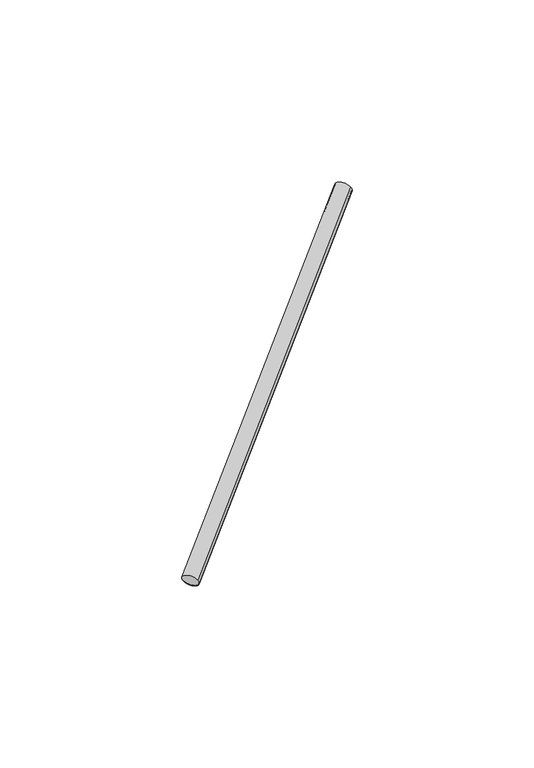
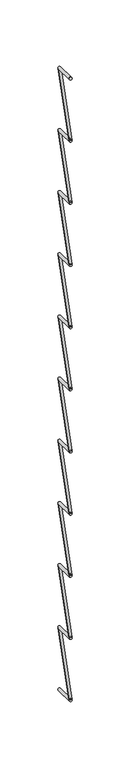
"""IFC4 building model written with IfcOpenShell, lengths in millimetres: proxy geometry, Pre-fab. (Vigota 2 - Pano 4)."""

from ifc_helpers import new_model, si_unit, point, frame, origin, origin_2d, place, context, project, spatial, circle_curve, trimmed, segment, composite_curve, outline, extrude, source, transform, mapped, element, save


def structural_framing_d21f35b0(model_context):
    return source(origin(), model_context, "Body", "SweptSolid", [
        extrude(outline(composite_curve([segment(trimmed(circle_curve(origin_2d(), 2.5), [point((2.5, 0.0))], [point((-2.5, 0.0))], False, "CARTESIAN"), True, "CONTINUOUS"), segment(trimmed(circle_curve(origin_2d(), 2.5), [point((-2.5, 0.0))], [point((2.5, 0.0))], False, "CARTESIAN"), True, "CONTINUOUS")], self_intersect=False)), frame((-42.0, 108.0, 1797.0), z_axis=(-0.3218603428886276, -0.8276408817707567, 0.4598004898837537), x_axis=(0.8192319205108605, 3.936835275445103e-11, 0.5734623443750141)), (0.0, 0.0, 1.0), 130.491379),
        extrude(outline(composite_curve([segment(trimmed(circle_curve(origin_2d(), 2.5), [point((2.5, 0.0))], [point((-2.5, 0.0))], False, "CARTESIAN"), True, "CONTINUOUS"), segment(trimmed(circle_curve(origin_2d(), 2.5), [point((-2.5, 0.0))], [point((2.5, 0.0))], False, "CARTESIAN"), True, "CONTINUOUS")], self_intersect=False)), frame((-84.0, 0.0, 1857.0), z_axis=(0.3218603428886276, 0.8276408817707567, 0.4598004898837537), x_axis=(0.8192319205108605, 3.936835275445103e-11, -0.5734623443750141)), (0.0, 0.0, 1.0), 130.491379),
        extrude(outline(composite_curve([segment(trimmed(circle_curve(origin_2d(), 2.5), [point((2.5, 0.0))], [point((-2.5, 0.0))], False, "CARTESIAN"), True, "CONTINUOUS"), segment(trimmed(circle_curve(origin_2d(), 2.5), [point((-2.5, 0.0))], [point((2.5, 0.0))], False, "CARTESIAN"), True, "CONTINUOUS")], self_intersect=False)), frame((-42.0, 108.0, 1917.0), z_axis=(-0.3218603428886276, -0.8276408817707567, 0.4598004898837537), x_axis=(0.8192319205108605, 3.936835275445103e-11, 0.5734623443750141)), (0.0, 0.0, 1.0), 130.491379),
        extrude(outline(composite_curve([segment(trimmed(circle_curve(origin_2d(), 2.5), [point((2.5, 0.0))], [point((-2.5, 0.0))], False, "CARTESIAN"), True, "CONTINUOUS"), segment(trimmed(circle_curve(origin_2d(), 2.5), [point((-2.5, 0.0))], [point((2.5, 0.0))], False, "CARTESIAN"), True, "CONTINUOUS")], self_intersect=False)), frame((-84.0, 0.0, 1977.0), z_axis=(0.3218603428886276, 0.8276408817707567, 0.4598004898837537), x_axis=(0.8192319205108605, 3.936835275445103e-11, -0.5734623443750141)), (0.0, 0.0, 1.0), 130.491379),
        extrude(outline(composite_curve([segment(trimmed(circle_curve(origin_2d(), 2.5), [point((2.5, 0.0))], [point((-2.5, 0.0))], False, "CARTESIAN"), True, "CONTINUOUS"), segment(trimmed(circle_curve(origin_2d(), 2.5), [point((-2.5, 0.0))], [point((2.5, 0.0))], False, "CARTESIAN"), True, "CONTINUOUS")], self_intersect=False)), frame((-42.0, 108.0, 2037.0), z_axis=(-0.3218603428886276, -0.8276408817707567, 0.4598004898837537), x_axis=(0.8192319205108605, 3.936835275445103e-11, 0.5734623443750141)), (0.0, 0.0, 1.0), 130.491379),
        extrude(outline(composite_curve([segment(trimmed(circle_curve(origin_2d(), 2.5), [point((2.5, 0.0))], [point((-2.5, 0.0))], False, "CARTESIAN"), True, "CONTINUOUS"), segment(trimmed(circle_curve(origin_2d(), 2.5), [point((-2.5, 0.0))], [point((2.5, 0.0))], False, "CARTESIAN"), True, "CONTINUOUS")], self_intersect=False)), frame((-84.0, 0.0, 2097.0), z_axis=(0.3218603428886276, 0.8276408817707567, 0.4598004898837537), x_axis=(0.8192319205108605, 3.936835275445103e-11, -0.5734623443750141)), (0.0, 0.0, 1.0), 130.491379),
        extrude(outline(composite_curve([segment(trimmed(circle_curve(origin_2d(), 2.5), [point((2.5, 0.0))], [point((-2.5, 0.0))], False, "CARTESIAN"), True, "CONTINUOUS"), segment(trimmed(circle_curve(origin_2d(), 2.5), [point((-2.5, 0.0))], [point((2.5, 0.0))], False, "CARTESIAN"), True, "CONTINUOUS")], self_intersect=False)), frame((-42.0, 108.0, 2157.0), z_axis=(-0.3218603428886276, -0.8276408817707567, 0.4598004898837537), x_axis=(0.8192319205108605, 3.936835275445103e-11, 0.5734623443750141)), (0.0, 0.0, 1.0), 130.491379),
        extrude(outline(composite_curve([segment(trimmed(circle_curve(origin_2d(), 2.5), [point((2.5, 0.0))], [point((-2.5, 0.0))], False, "CARTESIAN"), True, "CONTINUOUS"), segment(trimmed(circle_curve(origin_2d(), 2.5), [point((-2.5, 0.0))], [point((2.5, 0.0))], False, "CARTESIAN"), True, "CONTINUOUS")], self_intersect=False)), frame((-84.0, 0.0, 2217.0), z_axis=(0.3218603428886276, 0.8276408817707567, 0.4598004898837537), x_axis=(0.8192319205108605, 3.936835275445103e-11, -0.5734623443750141)), (0.0, 0.0, 1.0), 130.491379),
        extrude(outline(composite_curve([segment(trimmed(circle_curve(origin_2d(), 2.5), [point((2.5, 0.0))], [point((-2.5, 0.0))], False, "CARTESIAN"), True, "CONTINUOUS"), segment(trimmed(circle_curve(origin_2d(), 2.5), [point((-2.5, 0.0))], [point((2.5, 0.0))], False, "CARTESIAN"), True, "CONTINUOUS")], self_intersect=False)), frame((-42.0, 108.0, 2277.0), z_axis=(-0.3218603428886276, -0.8276408817707567, 0.4598004898837537), x_axis=(0.8192319205108605, 3.936835275445103e-11, 0.5734623443750141)), (0.0, 0.0, 1.0), 130.491379),
        extrude(outline(composite_curve([segment(trimmed(circle_curve(origin_2d(), 2.5), [point((2.5, 0.0))], [point((-2.5, 0.0))], False, "CARTESIAN"), True, "CONTINUOUS"), segment(trimmed(circle_curve(origin_2d(), 2.5), [point((-2.5, 0.0))], [point((2.5, 0.0))], False, "CARTESIAN"), True, "CONTINUOUS")], self_intersect=False)), frame((-84.0, 0.0, 2337.0), z_axis=(0.3218603428886276, 0.8276408817707567, 0.4598004898837537), x_axis=(0.8192319205108605, 3.936835275445103e-11, -0.5734623443750141)), (0.0, 0.0, 1.0), 130.491379),
        extrude(outline(composite_curve([segment(trimmed(circle_curve(origin_2d(), 2.5), [point((2.5, 0.0))], [point((-2.5, 0.0))], False, "CARTESIAN"), True, "CONTINUOUS"), segment(trimmed(circle_curve(origin_2d(), 2.5), [point((-2.5, 0.0))], [point((2.5, 0.0))], False, "CARTESIAN"), True, "CONTINUOUS")], self_intersect=False)), frame((-42.0, 108.0, 2397.0), z_axis=(-0.3218603428886276, -0.8276408817707567, 0.4598004898837537), x_axis=(0.8192319205108605, 3.936835275445103e-11, 0.5734623443750141)), (0.0, 0.0, 1.0), 130.491379),
        extrude(outline(composite_curve([segment(trimmed(circle_curve(origin_2d(), 2.5), [point((2.5, 0.0))], [point((-2.5, 0.0))], False, "CARTESIAN"), True, "CONTINUOUS"), segment(trimmed(circle_curve(origin_2d(), 2.5), [point((-2.5, 0.0))], [point((2.5, 0.0))], False, "CARTESIAN"), True, "CONTINUOUS")], self_intersect=False)), frame((-84.0, 0.0, 2457.0), z_axis=(0.3218603428886276, 0.8276408817707567, 0.4598004898837537), x_axis=(0.8192319205108605, 3.936835275445103e-11, -0.5734623443750141)), (0.0, 0.0, 1.0), 130.491379),
        extrude(outline(composite_curve([segment(trimmed(circle_curve(origin_2d(), 2.5), [point((2.5, 0.0))], [point((-2.5, 0.0))], False, "CARTESIAN"), True, "CONTINUOUS"), segment(trimmed(circle_curve(origin_2d(), 2.5), [point((-2.5, 0.0))], [point((2.5, 0.0))], False, "CARTESIAN"), True, "CONTINUOUS")], self_intersect=False)), frame((-42.0, 108.0, 2517.0), z_axis=(-0.3218603428886276, -0.8276408817707567, 0.4598004898837537), x_axis=(0.8192319205108605, 3.936835275445103e-11, 0.5734623443750141)), (0.0, 0.0, 1.0), 130.491379),
        extrude(outline(composite_curve([segment(trimmed(circle_curve(origin_2d(), 2.5), [point((2.5, 0.0))], [point((-2.5, 0.0))], False, "CARTESIAN"), True, "CONTINUOUS"), segment(trimmed(circle_curve(origin_2d(), 2.5), [point((-2.5, 0.0))], [point((2.5, 0.0))], False, "CARTESIAN"), True, "CONTINUOUS")], self_intersect=False)), frame((-84.0, 0.0, 2577.0), z_axis=(0.3218603428886276, 0.8276408817707567, 0.4598004898837537), x_axis=(0.8192319205108605, 3.936835275445103e-11, -0.5734623443750141)), (0.0, 0.0, 1.0), 130.491379),
        extrude(outline(composite_curve([segment(trimmed(circle_curve(origin_2d(), 2.5), [point((2.5, 0.0))], [point((-2.5, 0.0))], False, "CARTESIAN"), True, "CONTINUOUS"), segment(trimmed(circle_curve(origin_2d(), 2.5), [point((-2.5, 0.0))], [point((2.5, 0.0))], False, "CARTESIAN"), True, "CONTINUOUS")], self_intersect=False)), frame((-42.0, 108.0, 2637.0), z_axis=(-0.3218603428886276, -0.8276408817707567, 0.4598004898837537), x_axis=(0.8192319205108605, 3.936835275445103e-11, 0.5734623443750141)), (0.0, 0.0, 1.0), 130.491379),
        extrude(outline(composite_curve([segment(trimmed(circle_curve(origin_2d(), 2.5), [point((2.5, 0.0))], [point((-2.5, 0.0))], False, "CARTESIAN"), True, "CONTINUOUS"), segment(trimmed(circle_curve(origin_2d(), 2.5), [point((-2.5, 0.0))], [point((2.5, 0.0))], False, "CARTESIAN"), True, "CONTINUOUS")], self_intersect=False)), frame((-84.0, 0.0, 2697.0), z_axis=(0.3218603428886276, 0.8276408817707567, 0.4598004898837537), x_axis=(0.8192319205108605, 3.936835275445103e-11, -0.5734623443750141)), (0.0, 0.0, 1.0), 130.491379),
        extrude(outline(composite_curve([segment(trimmed(circle_curve(origin_2d(), 2.5), [point((2.5, 0.0))], [point((-2.5, 0.0))], False, "CARTESIAN"), True, "CONTINUOUS"), segment(trimmed(circle_curve(origin_2d(), 2.5), [point((-2.5, 0.0))], [point((2.5, 0.0))], False, "CARTESIAN"), True, "CONTINUOUS")], self_intersect=False)), frame((-42.0, 108.0, 2757.0), z_axis=(-0.3218603428886276, -0.8276408817707567, 0.4598004898837537), x_axis=(0.8192319205108605, 3.936835275445103e-11, 0.5734623443750141)), (0.0, 0.0, 1.0), 130.491379),
        extrude(outline(composite_curve([segment(trimmed(circle_curve(origin_2d(), 2.5), [point((2.5, 0.0))], [point((-2.5, 0.0))], False, "CARTESIAN"), True, "CONTINUOUS"), segment(trimmed(circle_curve(origin_2d(), 2.5), [point((-2.5, 0.0))], [point((2.5, 0.0))], False, "CARTESIAN"), True, "CONTINUOUS")], self_intersect=False)), frame((-84.0, 0.0, 2817.0), z_axis=(0.3218603428886276, 0.8276408817707567, 0.4598004898837537), x_axis=(0.8192319205108605, 3.936835275445103e-11, -0.5734623443750141)), (0.0, 0.0, 1.0), 130.491379),
        extrude(outline(composite_curve([segment(trimmed(circle_curve(origin_2d(), 2.5), [point((2.5, 0.0))], [point((-2.5, 0.0))], False, "CARTESIAN"), True, "CONTINUOUS"), segment(trimmed(circle_curve(origin_2d(), 2.5), [point((-2.5, 0.0))], [point((2.5, 0.0))], False, "CARTESIAN"), True, "CONTINUOUS")], self_intersect=False)), frame((-42.0, 108.0, 2877.0), z_axis=(-0.3218603428886276, -0.8276408817707567, 0.4598004898837537), x_axis=(0.8192319205108605, 3.936835275445103e-11, 0.5734623443750141)), (0.0, 0.0, 1.0), 130.491379),
        extrude(outline(composite_curve([segment(trimmed(circle_curve(origin_2d(), 2.5), [point((2.5, 0.0))], [point((-2.5, 0.0))], False, "CARTESIAN"), True, "CONTINUOUS"), segment(trimmed(circle_curve(origin_2d(), 2.5), [point((-2.5, 0.0))], [point((2.5, 0.0))], False, "CARTESIAN"), True, "CONTINUOUS")], self_intersect=False)), frame((-84.0, 0.0, 2937.0), z_axis=(0.3218603428886276, 0.8276408817707567, 0.4598004898837537), x_axis=(0.8192319205108605, 3.936835275445103e-11, -0.5734623443750141)), (0.0, 0.0, 1.0), 130.491379),
        extrude(outline(composite_curve([segment(trimmed(circle_curve(origin_2d(), 2.5), [point((2.5, 0.0))], [point((-2.5, 0.0))], False, "CARTESIAN"), True, "CONTINUOUS"), segment(trimmed(circle_curve(origin_2d(), 2.5), [point((-2.5, 0.0))], [point((2.5, 0.0))], False, "CARTESIAN"), True, "CONTINUOUS")], self_intersect=False)), frame((-42.0, 108.0, 2997.0), z_axis=(-0.3218603428886276, -0.8276408817707567, 0.4598004898837537), x_axis=(0.8192319205108605, 3.936835275445103e-11, 0.5734623443750141)), (0.0, 0.0, 1.0), 130.491379),
    ])


if __name__ == "__main__":
    model = new_model("IFC4")
    model_context = context("Model", 3, world=origin())
    ifc_project = project(units=[si_unit("LENGTHUNIT", "METRE", prefix="MILLI")], contexts=[model_context])
    site = spatial("IfcSite", under=ifc_project)
    building = spatial("IfcBuilding", under=site)
    placement = place(None, origin())
    structural_framing_shape = structural_framing_d21f35b0(model_context)
    element("IfcBuildingElementProxy", 1, Name="Pre-fab. (Vigota 2 - Pano 4)", ObjectType="Pre-fab. (Vigota 2 - Pano 4)", at=placement, inside=building, context=model_context, shape_type="MappedRepresentation", body=[
        mapped(structural_framing_shape, transform((0.0, 0.0, 0.0), x_axis=(1.0, 0.0, 0.0), y_axis=(0.0, 1.0, 0.0), z_axis=(0.0, 0.0, 1.0))),
    ])
    save(model, "model.ifc")

# Revit data of these elements
# Element 1 (IfcBuildingElementProxy, "Pre-fab. (Vigota 2 - Pano 4)")
#   Materials on its faces: "Aço"
# Materials
#   "Aço": class "Metal", colour RGB 120 120 120, transparency 0, Description = "Aço estrutural A36 grau, ASTM B, acabamento laminado", Cost = 0
